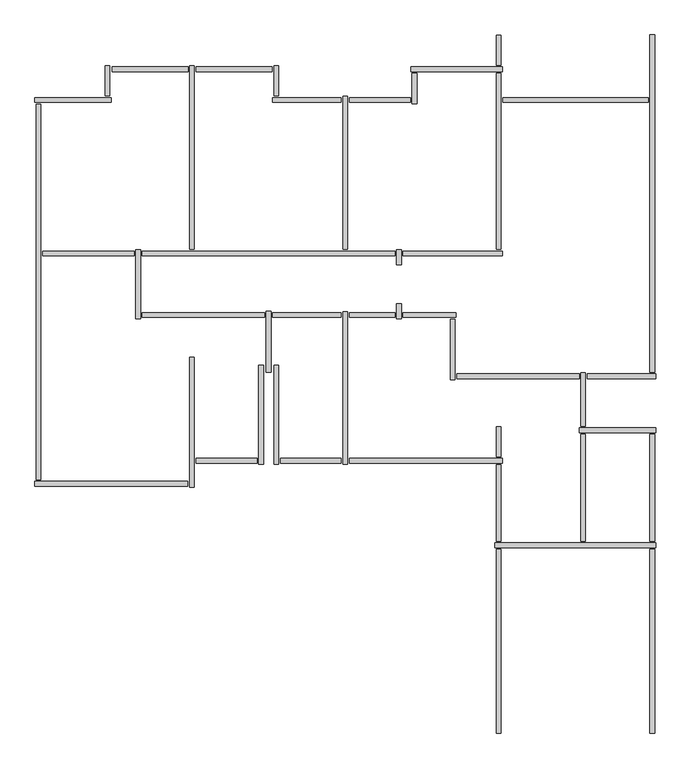
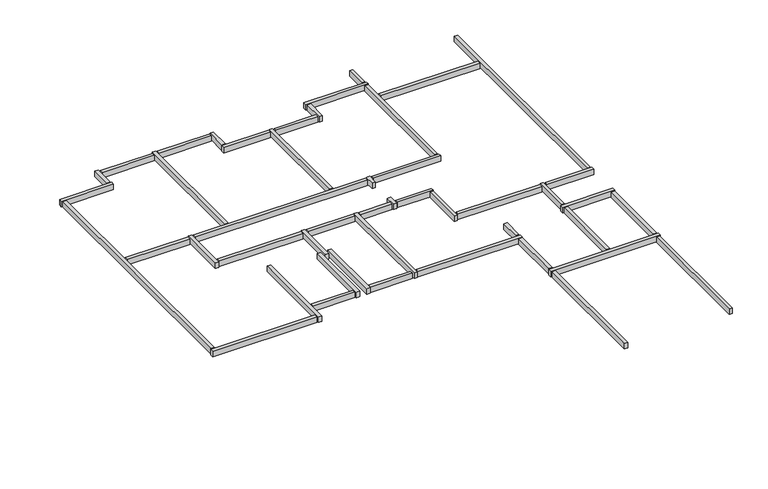
"""IFC4 building model written with IfcOpenShell, lengths in millimetres: beam geometry, Graute viga de respaldo15 : Graute viga de respaldo."""

from ifc_helpers import new_model, si_unit, frame, origin, place, context, project, spatial, polyline, outline, extrude, source, transform, mapped, element, save


def beam_dda22d07(model_context):
    return source(origin(), model_context, "Body", "SweptSolid", [
        extrude(outline(polyline([(-70718.7587292, 62785.4278788), (-70624.7587292, 62785.4278788), (-70624.7587292, 59195.4278788), (-70718.7587292, 59195.4278788), (-70718.7587292, 62785.4278788)])), frame((0.0, 0.0, 11632.9999999), z_axis=(0.0, 0.0, 1.0), x_axis=(1.0, 0.0, 0.0)), (0.0, 0.0, 1.0), 167.0),
        extrude(outline(polyline([(-67718.7587292, 62785.4278788), (-67624.7587292, 62785.4278788), (-67624.7587292, 59195.4278788), (-67718.7587292, 59195.4278788), (-67718.7587292, 62785.4278788)])), frame((0.0, 0.0, 11632.9999999), z_axis=(0.0, 0.0, 1.0), x_axis=(1.0, 0.0, 0.0)), (0.0, 0.0, 1.0), 167.0),
        extrude(outline(polyline([(-75401.7587292, 64562.4278788), (-75401.7587292, 64468.4278788), (-76591.7587292, 64468.4278788), (-76591.7587292, 64562.4278788), (-75401.7587292, 64562.4278788)])), frame((0.0, 0.0, 11632.9999999), z_axis=(0.0, 0.0, 1.0), x_axis=(1.0, 0.0, 0.0)), (0.0, 0.0, 1.0), 167.0),
        extrude(outline(polyline([(-73751.7587292, 64562.4278788), (-73751.7587292, 64468.4278788), (-74941.7587292, 64468.4278788), (-74941.7587292, 64562.4278788), (-73751.7587292, 64562.4278788)])), frame((0.0, 0.0, 11632.9999999), z_axis=(0.0, 0.0, 1.0), x_axis=(1.0, 0.0, 0.0)), (0.0, 0.0, 1.0), 167.0),
        extrude(outline(polyline([(-77801.7587292, 68612.4278788), (-77801.7587292, 68518.4278788), (-79591.7587292, 68518.4278788), (-79591.7587292, 68612.4278788), (-77801.7587292, 68612.4278788)])), frame((0.0, 0.0, 11632.9999999), z_axis=(0.0, 0.0, 1.0), x_axis=(1.0, 0.0, 0.0)), (0.0, 0.0, 1.0), 167.0),
        extrude(outline(polyline([(-72401.7587292, 71612.4278788), (-72401.7587292, 71518.4278788), (-73591.7587292, 71518.4278788), (-73591.7587292, 71612.4278788), (-72401.7587292, 71612.4278788)])), frame((0.0, 0.0, 11632.9999999), z_axis=(0.0, 0.0, 1.0), x_axis=(1.0, 0.0, 0.0)), (0.0, 0.0, 1.0), 167.0),
        extrude(outline(polyline([(-72274.7587292, 71495.4278788), (-72368.7587292, 71495.4278788), (-72368.7587292, 72085.4278788), (-72274.7587292, 72085.4278788), (-72274.7587292, 71495.4278788)])), frame((0.0, 0.0, 11632.9999999), z_axis=(0.0, 0.0, 1.0), x_axis=(1.0, 0.0, 0.0)), (0.0, 0.0, 1.0), 167.0),
        extrude(outline(polyline([(-70601.7587292, 72212.4278788), (-70601.7587292, 72118.4278788), (-72391.7587292, 72118.4278788), (-72391.7587292, 72212.4278788), (-70601.7587292, 72212.4278788)])), frame((0.0, 0.0, 11632.9999999), z_axis=(0.0, 0.0, 1.0), x_axis=(1.0, 0.0, 0.0)), (0.0, 0.0, 1.0), 167.0),
        extrude(outline(polyline([(-72668.7587292, 68635.4278788), (-72574.7587292, 68635.4278788), (-72574.7587292, 68345.4278788), (-72668.7587292, 68345.4278788), (-72668.7587292, 68635.4278788)])), frame((0.0, 0.0, 11632.9999999), z_axis=(0.0, 0.0, 1.0), x_axis=(1.0, 0.0, 0.0)), (0.0, 0.0, 1.0), 167.0),
        extrude(outline(polyline([(-75251.7587292, 67412.4278788), (-75251.7587292, 67318.4278788), (-77641.7587292, 67318.4278788), (-77641.7587292, 67412.4278788), (-75251.7587292, 67412.4278788)])), frame((0.0, 0.0, 11632.9999999), z_axis=(0.0, 0.0, 1.0), x_axis=(1.0, 0.0, 0.0)), (0.0, 0.0, 1.0), 167.0),
        extrude(outline(polyline([(-73751.7587292, 67412.4278788), (-73751.7587292, 67318.4278788), (-75091.7587292, 67318.4278788), (-75091.7587292, 67412.4278788), (-73751.7587292, 67412.4278788)])), frame((0.0, 0.0, 11632.9999999), z_axis=(0.0, 0.0, 1.0), x_axis=(1.0, 0.0, 0.0)), (0.0, 0.0, 1.0), 167.0),
        extrude(outline(polyline([(-72701.7587292, 67412.4278788), (-72701.7587292, 67318.4278788), (-73591.7587292, 67318.4278788), (-73591.7587292, 67412.4278788), (-72701.7587292, 67412.4278788)])), frame((0.0, 0.0, 11632.9999999), z_axis=(0.0, 0.0, 1.0), x_axis=(1.0, 0.0, 0.0)), (0.0, 0.0, 1.0), 167.0),
        extrude(outline(polyline([(-72668.7587292, 67585.4278788), (-72574.7587292, 67585.4278788), (-72574.7587292, 67295.4278788), (-72668.7587292, 67295.4278788), (-72668.7587292, 67585.4278788)])), frame((0.0, 0.0, 11632.9999999), z_axis=(0.0, 0.0, 1.0), x_axis=(1.0, 0.0, 0.0)), (0.0, 0.0, 1.0), 167.0),
        extrude(outline(polyline([(-71511.7587292, 67412.4278788), (-71511.7587292, 67318.4278788), (-72541.7587292, 67318.4278788), (-72541.7587292, 67412.4278788), (-71511.7587292, 67412.4278788)])), frame((0.0, 0.0, 11632.9999999), z_axis=(0.0, 0.0, 1.0), x_axis=(1.0, 0.0, 0.0)), (0.0, 0.0, 1.0), 167.0),
        extrude(outline(polyline([(-71524.7587292, 66095.4278788), (-71618.7587292, 66095.4278788), (-71618.7587292, 67285.4278788), (-71524.7587292, 67285.4278788), (-71524.7587292, 66095.4278788)])), frame((0.0, 0.0, 11632.9999999), z_axis=(0.0, 0.0, 1.0), x_axis=(1.0, 0.0, 0.0)), (0.0, 0.0, 1.0), 167.0),
        extrude(outline(polyline([(-69091.7587292, 66212.4278788), (-69091.7587292, 66118.4278788), (-71491.7587292, 66118.4278788), (-71491.7587292, 66212.4278788), (-69091.7587292, 66212.4278788)])), frame((0.0, 0.0, 11632.9999999), z_axis=(0.0, 0.0, 1.0), x_axis=(1.0, 0.0, 0.0)), (0.0, 0.0, 1.0), 167.0),
        extrude(outline(polyline([(-73718.7587292, 67430.4278788), (-73624.7587292, 67430.4278788), (-73624.7587292, 64445.4278788), (-73718.7587292, 64445.4278788), (-73718.7587292, 67430.4278788)])), frame((0.0, 0.0, 11632.9999999), z_axis=(0.0, 0.0, 1.0), x_axis=(1.0, 0.0, 0.0)), (0.0, 0.0, 1.0), 167.0),
        extrude(outline(polyline([(-70601.7587292, 64562.4278788), (-70601.7587292, 64468.4278788), (-73591.7587292, 64468.4278788), (-73591.7587292, 64562.4278788), (-70601.7587292, 64562.4278788)])), frame((0.0, 0.0, 11632.9999999), z_axis=(0.0, 0.0, 1.0), x_axis=(1.0, 0.0, 0.0)), (0.0, 0.0, 1.0), 167.0),
        extrude(outline(polyline([(-70718.7587292, 65185.4278788), (-70624.7587292, 65185.4278788), (-70624.7587292, 64595.4278788), (-70718.7587292, 64595.4278788), (-70718.7587292, 65185.4278788)])), frame((0.0, 0.0, 11632.9999999), z_axis=(0.0, 0.0, 1.0), x_axis=(1.0, 0.0, 0.0)), (0.0, 0.0, 1.0), 167.0),
        extrude(outline(polyline([(-70624.7587292, 62945.4278788), (-70718.7587292, 62945.4278788), (-70718.7587292, 64435.4278788), (-70624.7587292, 64435.4278788), (-70624.7587292, 62945.4278788)])), frame((0.0, 0.0, 11632.9999999), z_axis=(0.0, 0.0, 1.0), x_axis=(1.0, 0.0, 0.0)), (0.0, 0.0, 1.0), 167.0),
        extrude(outline(polyline([(-67624.7587292, 62945.4278788), (-67718.7587292, 62945.4278788), (-67718.7587292, 65035.4278788), (-67624.7587292, 65035.4278788), (-67624.7587292, 62945.4278788)])), frame((0.0, 0.0, 11632.9999999), z_axis=(0.0, 0.0, 1.0), x_axis=(1.0, 0.0, 0.0)), (0.0, 0.0, 1.0), 167.0),
        extrude(outline(polyline([(-68974.7587292, 62945.4278788), (-69068.7587292, 62945.4278788), (-69068.7587292, 65035.4278788), (-68974.7587292, 65035.4278788), (-68974.7587292, 62945.4278788)])), frame((0.0, 0.0, 11632.9999999), z_axis=(0.0, 0.0, 1.0), x_axis=(1.0, 0.0, 0.0)), (0.0, 0.0, 1.0), 167.0),
        extrude(outline(polyline([(-69068.7587292, 66235.4278788), (-68974.7587292, 66235.4278788), (-68974.7587292, 65195.4278788), (-69068.7587292, 65195.4278788), (-69068.7587292, 66235.4278788)])), frame((0.0, 0.0, 11632.9999999), z_axis=(0.0, 0.0, 1.0), x_axis=(1.0, 0.0, 0.0)), (0.0, 0.0, 1.0), 167.0),
        extrude(outline(polyline([(-67751.7587292, 71612.4278788), (-67751.7587292, 71518.4278788), (-70591.7587292, 71518.4278788), (-70591.7587292, 71612.4278788), (-67751.7587292, 71612.4278788)])), frame((0.0, 0.0, 11632.9999999), z_axis=(0.0, 0.0, 1.0), x_axis=(1.0, 0.0, 0.0)), (0.0, 0.0, 1.0), 167.0),
        extrude(outline(polyline([(-70624.7587292, 68645.4278788), (-70718.7587292, 68645.4278788), (-70718.7587292, 72085.4278788), (-70624.7587292, 72085.4278788), (-70624.7587292, 68645.4278788)])), frame((0.0, 0.0, 11632.9999999), z_axis=(0.0, 0.0, 1.0), x_axis=(1.0, 0.0, 0.0)), (0.0, 0.0, 1.0), 167.0),
        extrude(outline(polyline([(-70601.7587292, 68612.4278788), (-70601.7587292, 68518.4278788), (-72541.7587292, 68518.4278788), (-72541.7587292, 68612.4278788), (-70601.7587292, 68612.4278788)])), frame((0.0, 0.0, 11632.9999999), z_axis=(0.0, 0.0, 1.0), x_axis=(1.0, 0.0, 0.0)), (0.0, 0.0, 1.0), 167.0),
        extrude(outline(polyline([(-72701.7587292, 68612.4278788), (-72701.7587292, 68518.4278788), (-77641.7587292, 68518.4278788), (-77641.7587292, 68612.4278788), (-72701.7587292, 68612.4278788)])), frame((0.0, 0.0, 11632.9999999), z_axis=(0.0, 0.0, 1.0), x_axis=(1.0, 0.0, 0.0)), (0.0, 0.0, 1.0), 167.0),
        extrude(outline(polyline([(-73718.7587292, 71635.4278788), (-73624.7587292, 71635.4278788), (-73624.7587292, 68645.4278788), (-73718.7587292, 68645.4278788), (-73718.7587292, 71635.4278788)])), frame((0.0, 0.0, 11632.9999999), z_axis=(0.0, 0.0, 1.0), x_axis=(1.0, 0.0, 0.0)), (0.0, 0.0, 1.0), 167.0),
        extrude(outline(polyline([(-75091.7587292, 71518.4278788), (-75091.7587292, 71612.4278788), (-73751.7587292, 71612.4278788), (-73751.7587292, 71518.4278788), (-75091.7587292, 71518.4278788)])), frame((0.0, 0.0, 11632.9999999), z_axis=(0.0, 0.0, 1.0), x_axis=(1.0, 0.0, 0.0)), (0.0, 0.0, 1.0), 167.0),
        extrude(outline(polyline([(-75068.7587292, 72235.4278788), (-74974.7587292, 72235.4278788), (-74974.7587292, 71645.4278788), (-75068.7587292, 71645.4278788), (-75068.7587292, 72235.4278788)])), frame((0.0, 0.0, 11632.9999999), z_axis=(0.0, 0.0, 1.0), x_axis=(1.0, 0.0, 0.0)), (0.0, 0.0, 1.0), 167.0),
        extrude(outline(polyline([(-75101.7587292, 72212.4278788), (-75101.7587292, 72118.4278788), (-76591.7587292, 72118.4278788), (-76591.7587292, 72212.4278788), (-75101.7587292, 72212.4278788)])), frame((0.0, 0.0, 11632.9999999), z_axis=(0.0, 0.0, 1.0), x_axis=(1.0, 0.0, 0.0)), (0.0, 0.0, 1.0), 167.0),
        extrude(outline(polyline([(-78230.736554, 72117.4278788), (-78230.736554, 72212.4278788), (-76741.7587292, 72212.4278788), (-76741.7587292, 72117.4278788), (-78230.736554, 72117.4278788)])), frame((0.0, 0.0, 11617.1856208), z_axis=(0.0, 0.0, 1.0), x_axis=(1.0, 0.0, 0.0)), (0.0, 0.0, 1.0), 165.0),
        extrude(outline(polyline([(-79624.7587292, 64145.4278788), (-79718.7587292, 64145.4278788), (-79718.7587292, 71485.4278788), (-79624.7587292, 71485.4278788), (-79624.7587292, 64145.4278788)])), frame((0.0, 0.0, 11632.9999999), z_axis=(0.0, 0.0, 1.0), x_axis=(1.0, 0.0, 0.0)), (0.0, 0.0, 1.0), 167.0),
        extrude(outline(polyline([(-77674.7587292, 67295.4278788), (-77768.7587292, 67295.4278788), (-77768.7587292, 68640.7810915), (-77674.7587292, 68640.7810915), (-77674.7587292, 67295.4278788)])), frame((0.0, 0.0, 11632.9999999), z_axis=(0.0, 0.0, 1.0), x_axis=(1.0, 0.0, 0.0)), (0.0, 0.0, 1.0), 167.0),
        extrude(outline(polyline([(-75124.7587292, 66245.4278788), (-75218.7587292, 66245.4278788), (-75218.7587292, 67435.4278788), (-75124.7587292, 67435.4278788), (-75124.7587292, 66245.4278788)])), frame((0.0, 0.0, 11632.9999999), z_axis=(0.0, 0.0, 1.0), x_axis=(1.0, 0.0, 0.0)), (0.0, 0.0, 1.0), 167.0),
        extrude(outline(polyline([(-75274.7587292, 64445.4278788), (-75368.7587292, 64445.4278788), (-75368.7587292, 66385.4278788), (-75274.7587292, 66385.4278788), (-75274.7587292, 64445.4278788)])), frame((0.0, 0.0, 11632.9999999), z_axis=(0.0, 0.0, 1.0), x_axis=(1.0, 0.0, 0.0)), (0.0, 0.0, 1.0), 167.0),
        extrude(outline(polyline([(-74974.7587292, 64445.4278788), (-75068.7587292, 64445.4278788), (-75068.7587292, 66385.4278788), (-74974.7587292, 66385.4278788), (-74974.7587292, 64445.4278788)])), frame((0.0, 0.0, 11632.9999999), z_axis=(0.0, 0.0, 1.0), x_axis=(1.0, 0.0, 0.0)), (0.0, 0.0, 1.0), 167.0),
        extrude(outline(polyline([(-76624.7587292, 63995.4278788), (-76718.7587292, 63995.4278788), (-76718.7587292, 66535.4278788), (-76624.7587292, 66535.4278788), (-76624.7587292, 63995.4278788)])), frame((0.0, 0.0, 11632.9999999), z_axis=(0.0, 0.0, 1.0), x_axis=(1.0, 0.0, 0.0)), (0.0, 0.0, 1.0), 167.0),
        extrude(outline(polyline([(-79741.7587292, 64018.4278788), (-79741.7587292, 64112.4278788), (-76751.7587292, 64112.4278788), (-76751.7587292, 64018.4278788), (-79741.7587292, 64018.4278788)])), frame((0.0, 0.0, 11632.9999999), z_axis=(0.0, 0.0, 1.0), x_axis=(1.0, 0.0, 0.0)), (0.0, 0.0, 1.0), 167.0),
        extrude(outline(polyline([(-78368.7587292, 72235.4278788), (-78274.7587292, 72235.4278788), (-78274.7587292, 71645.4278788), (-78368.7587292, 71645.4278788), (-78368.7587292, 72235.4278788)])), frame((0.0, 0.0, 11632.9999999), z_axis=(0.0, 0.0, 1.0), x_axis=(1.0, 0.0, 0.0)), (0.0, 0.0, 1.0), 167.0),
        extrude(outline(polyline([(-78251.7587292, 71612.4278788), (-78251.7587292, 71518.4278788), (-79741.7587292, 71518.4278788), (-79741.7587292, 71612.4278788), (-78251.7587292, 71612.4278788)])), frame((0.0, 0.0, 11632.9999999), z_axis=(0.0, 0.0, 1.0), x_axis=(1.0, 0.0, 0.0)), (0.0, 0.0, 1.0), 167.0),
        extrude(outline(polyline([(-76718.7587292, 72235.4278788), (-76624.7587292, 72235.4278788), (-76624.7587292, 68645.4278788), (-76718.7587292, 68645.4278788), (-76718.7587292, 72235.4278788)])), frame((0.0, 0.0, 11632.9999999), z_axis=(0.0, 0.0, 1.0), x_axis=(1.0, 0.0, 0.0)), (0.0, 0.0, 1.0), 167.0),
        extrude(outline(polyline([(-70718.7587292, 72835.4278788), (-70624.7587292, 72835.4278788), (-70624.7587292, 72245.4278788), (-70718.7587292, 72245.4278788), (-70718.7587292, 72835.4278788)])), frame((0.0, 0.0, 11632.9999999), z_axis=(0.0, 0.0, 1.0), x_axis=(1.0, 0.0, 0.0)), (0.0, 0.0, 1.0), 167.0),
        extrude(outline(polyline([(-67601.7587292, 65162.4278788), (-67601.7587292, 65068.4278788), (-69091.7587292, 65068.4278788), (-69091.7587292, 65162.4278788), (-67601.7587292, 65162.4278788)])), frame((0.0, 0.0, 11632.9999999), z_axis=(0.0, 0.0, 1.0), x_axis=(1.0, 0.0, 0.0)), (0.0, 0.0, 1.0), 167.0),
        extrude(outline(polyline([(-67601.7587292, 62912.4278788), (-67601.7587292, 62818.4278788), (-70741.7587292, 62818.4278788), (-70741.7587292, 62912.4278788), (-67601.7587292, 62912.4278788)])), frame((0.0, 0.0, 11632.9999999), z_axis=(0.0, 0.0, 1.0), x_axis=(1.0, 0.0, 0.0)), (0.0, 0.0, 1.0), 167.0),
        extrude(outline(polyline([(-67601.7587292, 66212.4278788), (-67601.7587292, 66118.4278788), (-68941.7587292, 66118.4278788), (-68941.7587292, 66212.4278788), (-67601.7587292, 66212.4278788)])), frame((0.0, 0.0, 11632.9999999), z_axis=(0.0, 0.0, 1.0), x_axis=(1.0, 0.0, 0.0)), (0.0, 0.0, 1.0), 167.0),
        extrude(outline(polyline([(-67718.7587292, 72837.9577736), (-67624.7587292, 72837.9577736), (-67624.7587292, 66245.4278788), (-67718.7587292, 66245.4278788), (-67718.7587292, 72837.9577736)])), frame((0.0, 0.0, 11632.9999999), z_axis=(0.0, 0.0, 1.0), x_axis=(1.0, 0.0, 0.0)), (0.0, 0.0, 1.0), 167.0),
    ])


if __name__ == "__main__":
    model = new_model("IFC4")
    model_context = context("Model", 3, world=origin())
    ifc_project = project(units=[si_unit("LENGTHUNIT", "METRE", prefix="MILLI")], contexts=[model_context])
    site = spatial("IfcSite", under=ifc_project)
    building = spatial("IfcBuilding", under=site)
    placement = place(None, origin())
    beam_shape = beam_dda22d07(model_context)
    element("IfcBeam", 1, ObjectType="Graute viga de respaldo15 : Graute viga de respaldo", at=placement, inside=building, context=model_context, shape_type="MappedRepresentation", body=[
        mapped(beam_shape, transform((0.0, 0.0, 0.0), x_axis=(1.0, 0.0, 0.0), y_axis=(0.0, 1.0, 0.0), z_axis=(0.0, 0.0, 1.0))),
    ])
    save(model, "model.ifc")

# Revit data of these elements
# Element 1 (IfcBeam, "Graute viga de respaldo15 : Graute viga de respaldo")
#   Materials on its faces: "Concreto, Faixa de areia/cimento"
# Materials
#   "Concreto, Faixa de areia/cimento": class "Concreto", colour RGB 127 127 127, transparency 0, Description = "Revestimento de laje de concreto", Cost = 0
